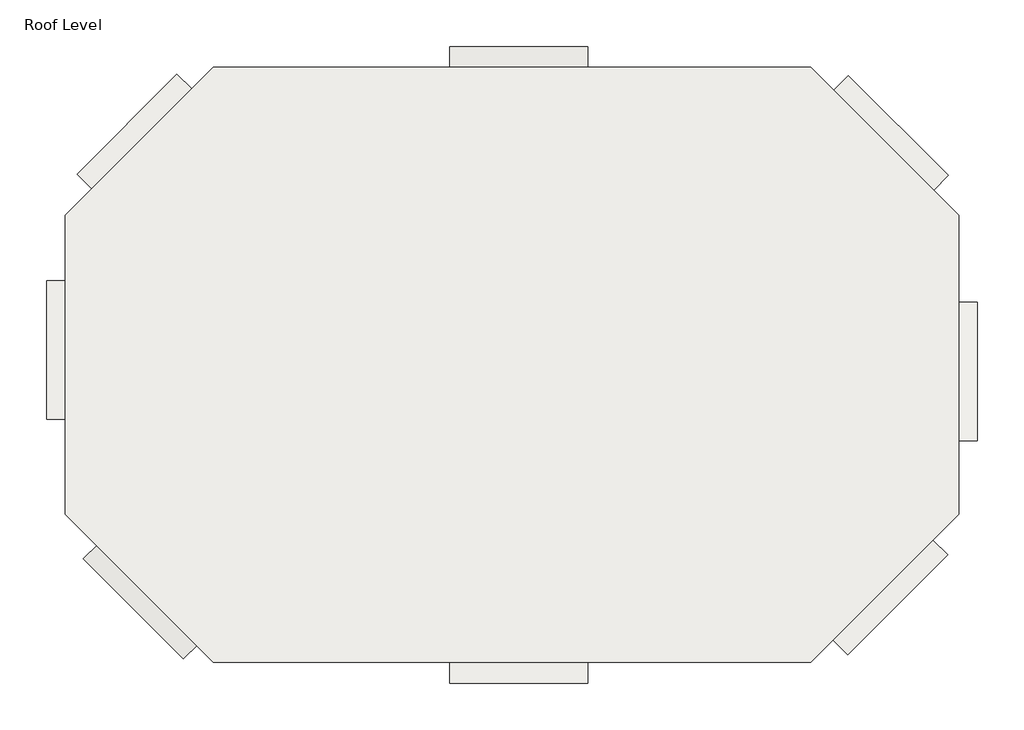
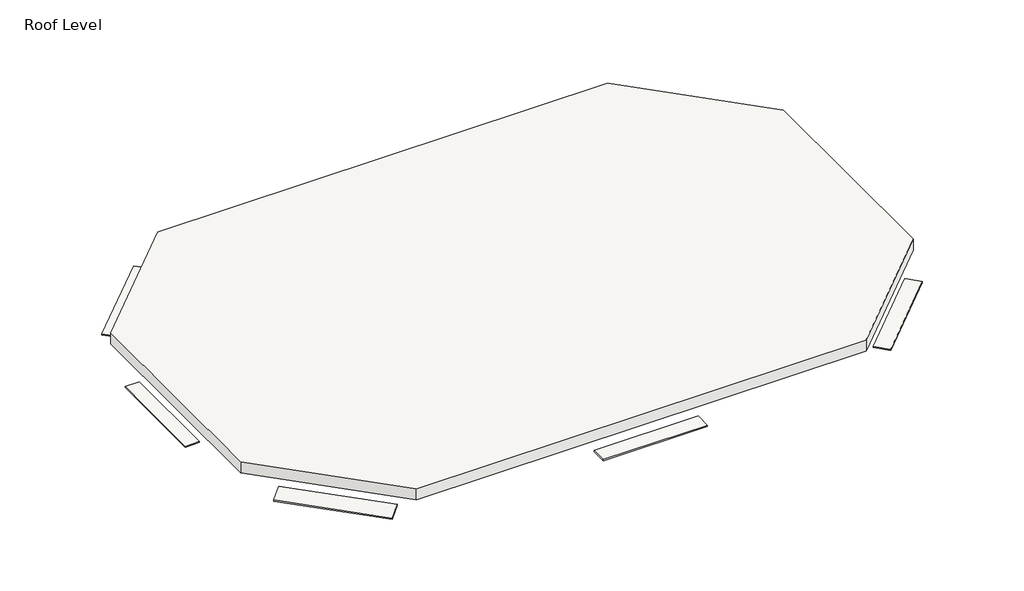
# One storey: 9 roofs.
"""IFC4 building model written with IfcOpenShell, lengths in millimetres."""

from ifc_helpers import new_model, si_unit, frame, origin, place, context, project, spatial, polyline, outline, extrude, element, save

model = new_model("IFC4")

# Units and contexts
model_context = context("Model", 3, world=origin())
ifc_project = project(units=[si_unit("LENGTHUNIT", "METRE", prefix="MILLI")], contexts=[model_context])

# Site, building, storey
site = spatial("IfcSite", under=ifc_project)
building = spatial("IfcBuilding", under=site)
storey = spatial("IfcBuildingStorey", under=building, Name="Roof Level", Elevation=7924.8)

# Roofs
placement = place(None, origin())
element("IfcRoof", 1, ObjectType="Generic - 125mm shading", at=placement, inside=storey, context=model_context, shape_type="SweptSolid", body=[
    extrude(outline(polyline([(18552.7836697, -8602.5147149), (23180.3836697, -8602.5147149), (23180.3836697, -9302.5147149), (18552.7836697, -9302.5147149), (18552.7836697, -8602.5147149)])), frame((0.0, 0.0, 7412.4), z_axis=(0.0, 0.0, 1.0), x_axis=(1.0, 0.0, 0.0)), (0.0, 0.0, 1.0), 50.0),
])
element("IfcRoof", 2, ObjectType="Generic - 125mm shading", at=placement, inside=storey, context=model_context, shape_type="SweptSolid", body=[
    extrude(outline(polyline([(11296.9802217, 7463.1713306), (11996.9802217, 7586.6002171), (11996.9802217, 7535.8288865), (11296.9802217, 7412.4), (11296.9802217, 7463.1713306)])), frame((18552.7836697, 0.0, 0.0), z_axis=(1.0, 0.0, 0.0), x_axis=(0.0, 1.0, 0.0)), (0.0, 0.0, 1.0), 4627.6),
])
element("IfcRoof", 3, ObjectType="Generic - 125mm shading", at=placement, inside=storey, context=model_context, shape_type="SweptSolid", body=[
    extrude(outline(polyline([(34745.7885808, 7190.4058824), (31403.3995039, 10532.7949592), (31895.6627273, 11025.0581826), (35238.0518042, 7682.6691057), (34745.7885808, 7190.4058824)])), frame((0.0, 0.0, 7362.4), z_axis=(0.0, 0.0, 1.0), x_axis=(1.0, 0.0, 0.0)), (0.0, 0.0, 1.0), 50.0),
])
element("IfcRoof", 4, ObjectType="Generic - 125mm shading", at=placement, inside=storey, context=model_context, shape_type="SweptSolid", body=[
    extrude(outline(polyline([(31379.6986616, -7862.0302949), (34722.0877385, -4519.641218), (35214.3509618, -5011.9044414), (31871.961885, -8354.2935183), (31379.6986616, -7862.0302949)])), frame((0.0, 0.0, 7362.4), z_axis=(0.0, 0.0, 1.0), x_axis=(1.0, 0.0, 0.0)), (0.0, 0.0, 1.0), 50.0),
])
element("IfcRoof", 5, ObjectType="Generic - 125mm shading", at=placement, inside=storey, context=model_context, shape_type="SweptSolid", body=[
    extrude(outline(polyline([(9921.2320547, 10578.9980348), (6578.8429778, 7236.6089579), (6086.5797544, 7728.8721813), (9428.9688313, 11071.2612582), (9921.2320547, 10578.9980348)])), frame((0.0, 0.0, 7362.4), z_axis=(0.0, 0.0, 1.0), x_axis=(1.0, 0.0, 0.0)), (0.0, 0.0, 1.0), 50.0),
])
element("IfcRoof", 6, ObjectType="Generic - 125mm shading", at=placement, inside=storey, context=model_context, shape_type="SweptSolid", body=[
    extrude(outline(polyline([(696.1653268, 410.636191), (0.0, 597.1731281), (0.0, 648.9369371), (696.1653268, 462.4), (696.1653268, 410.636191)])), frame((9643.8495861, -8489.3364797, 7924.8), z_axis=(-0.7071067811865483, 0.7071067811865468, 0.0), x_axis=(0.7071067811865468, 0.7071067811865483, 0.0)), (0.0, 0.0, 1.0), 4726.8519632),
])
element("IfcRoof", 7, ObjectType="Generic - 125mm shading", at=placement, inside=storey, context=model_context, shape_type="SweptSolid", body=[
    extrude(outline(polyline([(7353.17856, 36212.7617098), (7463.1713306, 35588.9617098), (7412.4, 35588.9617098), (7302.4072294, 36212.7617098), (7353.17856, 36212.7617098)])), frame((0.0, -1191.3598794, 0.0), z_axis=(0.0, 1.0, 0.0), x_axis=(0.0, 0.0, 1.0)), (0.0, 0.0, 1.0), 4627.6),
])
element("IfcRoof", 8, ObjectType="Generic - 125mm shading", at=placement, inside=storey, context=model_context, shape_type="SweptSolid", body=[
    extrude(outline(polyline([(5689.4667732, 4156.608734), (5689.4667732, -470.991266), (5065.6667732, -470.991266), (5065.6667732, 4156.608734), (5689.4667732, 4156.608734)])), frame((0.0, 0.0, 7412.4), z_axis=(0.0, 0.0, 1.0), x_axis=(1.0, 0.0, 0.0)), (0.0, 0.0, 1.0), 50.0),
])
element("IfcRoof", 9, ObjectType="Pitched - Warm - Industrial", at=placement, inside=storey, context=model_context, shape_type="SweptSolid", body=[
    extrude(outline(polyline([(5689.4667732, 6347.2327534), (10639.2142415, 11296.9802217), (30639.2142415, 11296.9802217), (35588.9617098, 6347.2327534), (35588.9617098, -3652.7672466), (30639.2142415, -8602.5147149), (10639.2142415, -8602.5147149), (5689.4667732, -3652.7672466), (5689.4667732, 6347.2327534)])), frame((0.0, 0.0, 7924.8), z_axis=(0.0, 0.0, 1.0), x_axis=(1.0, 0.0, 0.0)), (0.0, 0.0, 1.0), 515.0),
])

save(model, "model.ifc")

# Revit data of these elements
# Type "Generic - 125mm shading"
#   Layers, outside or top first: 50 mm no material (function 1)
# Type "Pitched - Warm - Industrial"
#   Layers, outside or top first: 50 mm "Roofing, Standing Seam" (function 5); 220 mm "Rigid insulation" (function 3); 20 mm "Metal Panel" (function 4); 225 mm "Steel Purlins" (function 1)
# Elements 1, 8 (IfcRoof, "Generic - 125mm shading")
#   built-in parameter 1001705 = 24.4829 (stored number, unit not read)
#   built-in parameter 1001701 = -1.6811 (stored number, unit not read)
#   built-in parameter 1001710 = 33615
#   Phase Created = New Construction
#   Materials on its faces: "Default Roof"
# Element 2 (IfcRoof, "Generic - 125mm shading")
#   built-in parameter 1001705 = 24.8904 (stored number, unit not read)
#   built-in parameter 1001701 = -1.6811 (stored number, unit not read)
#   built-in parameter 1001710 = 33615
#   Phase Created = New Construction
#   Materials on its faces: "Default Roof"
# Elements 3, 4, 5 (IfcRoof, "Generic - 125mm shading")
#   built-in parameter 1001705 = 24.3189 (stored number, unit not read)
#   built-in parameter 1001701 = -1.84514 (stored number, unit not read)
#   built-in parameter 1001710 = 33615
#   Phase Created = New Construction
#   Materials on its faces: "Default Roof"
# Element 6 (IfcRoof, "Generic - 125mm shading")
#   built-in parameter 1001705 = 24.6528 (stored number, unit not read)
#   built-in parameter 1001701 = -1.51706 (stored number, unit not read)
#   built-in parameter 1001710 = 33615
#   Phase Created = New Construction
#   Materials on its faces: "Default Roof"
# Element 7 (IfcRoof, "Generic - 125mm shading")
#   built-in parameter 1001705 = 24.4855 (stored number, unit not read)
#   built-in parameter 1001701 = -1.6811 (stored number, unit not read)
#   built-in parameter 1001710 = 33615
#   Phase Created = New Construction
#   Materials on its faces: "Default Roof"
# Element 9 (IfcRoof, "Pitched - Warm - Industrial")
#   built-in parameter 1001705 = 27.6896 (stored number, unit not read)
#   built-in parameter 1001710 = 33615
#   Phase Created = New Construction
#   Materials on its faces: "Steel Purlins", "Roofing, Standing Seam"
# Materials
#   "Roofing, Standing Seam": class "Metal", colour RGB 247 247 247, transparency 0, Description = "Aluminum standing seam roofing", Cost = 0
#   "Rigid insulation": class "Generic", colour RGB 127 127 127, transparency 0, Description = "Rigid foam insulation board", Cost = 0
#   "Metal Panel": class "Metal", colour RGB 247 247 247, transparency 0, Description = "Stainless steel panels", Cost = 0
#   "Steel Purlins": class "Metal", colour RGB 247 247 247, transparency 0, Description = "Light gauge steel purlins", Cost = 0
#   "Default Roof": class "Miscellaneous", colour RGB 0 127 0, transparency 0, Cost = 0
